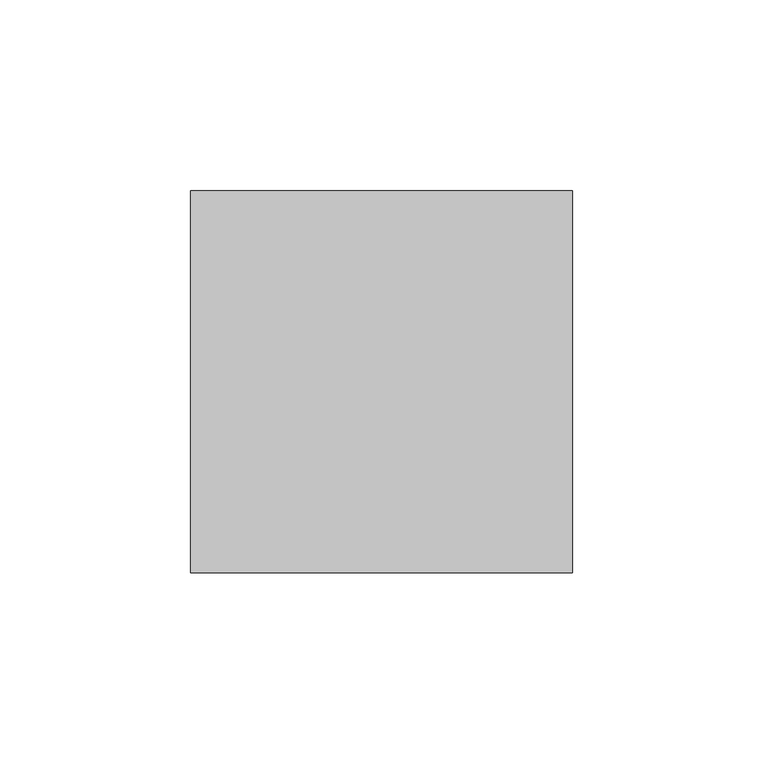
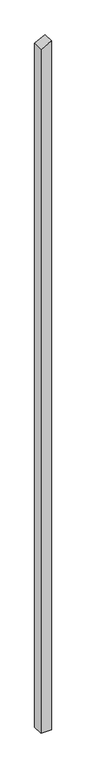
"""IFC4 building model written with IfcOpenShell, lengths in millimetres: column geometry, Holzstütze 159806 : Holzstütze 159806."""

from ifc_helpers import new_model, si_unit, frame, origin, place, context, project, spatial, polyline, outline, extrude, source, transform, mapped, element, save


def column_414bb659(model_context):
    return source(origin(), model_context, "Body", "SweptSolid", [
        extrude(outline(polyline([(-500.0, 157297.7593015), (-500.0, 157397.7593015), (6396.6643707, 157397.7593015), (6345.7118258, 157297.7593015), (-500.0, 157297.7593015)])), frame((0.0, 41761.7297978, 0.0), z_axis=(0.0, 1.0, 0.0), x_axis=(0.0, 0.0, 1.0)), (0.0, 0.0, 1.0), 100.0),
    ])


if __name__ == "__main__":
    model = new_model("IFC4")
    model_context = context("Model", 3, world=origin())
    ifc_project = project(units=[si_unit("LENGTHUNIT", "METRE", prefix="MILLI")], contexts=[model_context])
    site = spatial("IfcSite", under=ifc_project)
    building = spatial("IfcBuilding", under=site)
    placement = place(None, origin())
    column_shape = column_414bb659(model_context)
    element("IfcColumn", 1, ObjectType="Holzstütze 159806 : Holzstütze 159806", at=placement, inside=building, context=model_context, shape_type="MappedRepresentation", body=[
        mapped(column_shape, transform((0.0, 0.0, 0.0), x_axis=(1.0, 0.0, 0.0), y_axis=(0.0, 1.0, 0.0), z_axis=(0.0, 0.0, 1.0))),
    ])
    save(model, "model.ifc")

# Revit data of these elements
# Type "Holzstütze 159806 : Holzstütze 159806"
#   Abrechnungsart = "m"
#   Allright_Bauteil_ID = "0152St 0000143340"
#   Bezeichnung = "Holzstütze"
#   Codetext = "ST-HOLZ\\"
#   Gewerk = "Zimmer- und Holzbauarbeiten"
#   Material = "Holz"
#   Objektname = "Stütze"
#   NameOverride = "Holzstütze"
#   Reference = "Holzstütze"
#   Status = "NEW"
#   ThermalTransmittance = 0.0000 BTU/(h·ft²·°F)
#   Roll = 0.00°
#   Slope = 0.00°
#   2D Interaktion = yes
#   IsExternal = yes
#   LoadBearing = yes
# Element 1 (IfcColumn, "Holzstütze 159806 : Holzstütze 159806")
#   Materials on its faces: "holzschalung"
# Materials
#   "holzschalung": class "Unassigned", colour RGB 128 128 128, transparency 0
